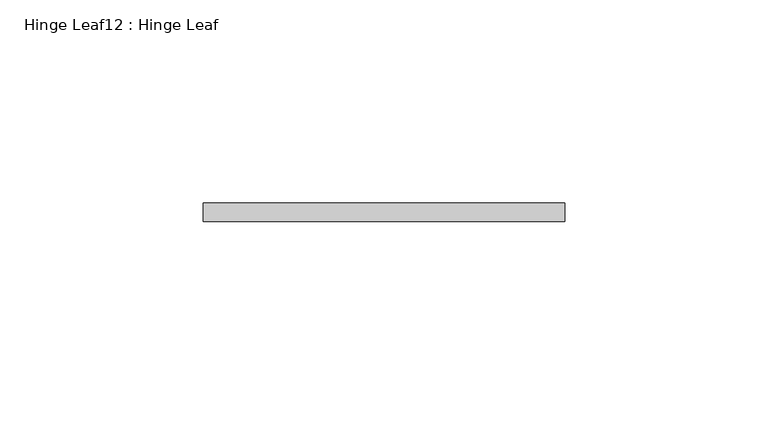
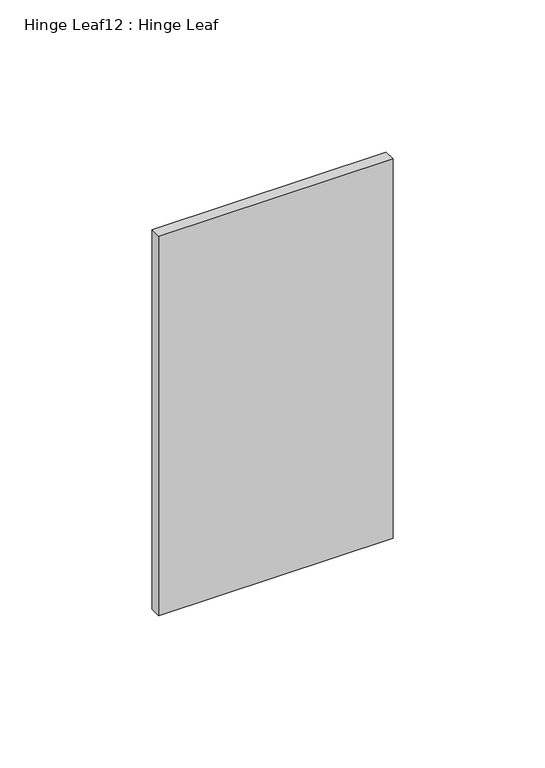
"""IFC4 building model written with IfcOpenShell, lengths in millimetres: proxy geometry, Hinge Leaf12 : Hinge Leaf."""

import ifcopenshell
import ifcopenshell.guid

model = None  # the IFC model being written
_history = None  # IfcOwnerHistory: only IFC2X3 demands one
_inside = {}  # id of a spatial element -> (the spatial element, [elements in it])
_under = {}  # id of a project, library or spatial element -> (it, [spatial elements below it])
_declared = {}  # id of a project -> (the project, [libraries it declares])
_typed = {}  # id of a type object -> (the type object, [elements of that type])
_made_of = {}  # id of a material, layer set ... -> (it, [elements and type objects made of it])


def new_model(schema):
    """Start an empty IFC model of exactly this schema.

    Asked for "IFC4X3", IfcOpenShell would pick the latest addendum, in which some entities
    have other attributes; the version numbers below select the first issue.
    IFC2X3 requires an IfcOwnerHistory on every rooted entity: one is made here for all.
    """
    global model, _history
    if schema == "IFC4X3":
        model = ifcopenshell.file(schema_version=(4, 3, 0, 0))
    else:
        model = ifcopenshell.file(schema=schema)
    _inside.clear()
    _under.clear()
    _declared.clear()
    _typed.clear()
    _made_of.clear()
    _history = None
    if model.schema == "IFC2X3":
        org = make("IfcOrganization", Name="unknown")
        user = make(
            "IfcPersonAndOrganization",
            ThePerson=make("IfcPerson", FamilyName="unknown"),
            TheOrganization=org,
        )
        app = make(
            "IfcApplication",
            ApplicationDeveloper=org,
            Version="unknown",
            ApplicationFullName="unknown",
            ApplicationIdentifier="unknown",
        )
        _history = make(
            "IfcOwnerHistory",
            OwningUser=user,
            OwningApplication=app,
            ChangeAction="ADDED",
            CreationDate=0,
        )
    return model


def make(cls, **values):
    """One entity of the class cls with the attributes given. An attribute that is None is left unset."""
    return model.create_entity(
        cls, **{name: value for name, value in values.items() if value is not None}
    )


def rooted(cls, **values):
    """An entity with a GlobalId (a new one), such as an element, a storey or a relation."""
    return make(cls, GlobalId=ifcopenshell.guid.new(), OwnerHistory=_history, **values)


def si_unit(unit_type, name, prefix=None):
    """IfcSIUnit, for example si_unit("LENGTHUNIT", "METRE", prefix="MILLI")."""
    return make("IfcSIUnit", UnitType=unit_type, Prefix=prefix, Name=name)


def assignment(units):
    """IfcUnitAssignment: the units of a project."""
    return None if units is None else make("IfcUnitAssignment", Units=units)


def point(xyz):
    """IfcCartesianPoint."""
    return None if xyz is None else make("IfcCartesianPoint", Coordinates=xyz)


def direction(xyz):
    """IfcDirection."""
    return None if xyz is None else make("IfcDirection", DirectionRatios=xyz)


def frame(location, z_axis=None, x_axis=None):
    """IfcAxis2Placement3D, a coordinate frame: its origin and axes. An axis left out is left unset."""
    return make(
        "IfcAxis2Placement3D",
        Location=point(location),
        Axis=direction(z_axis),
        RefDirection=direction(x_axis),
    )


def origin():
    """The frame at (0, 0, 0) with its axes left unset."""
    return frame((0.0, 0.0, 0.0))


def place(relative_to, where):
    """IfcLocalPlacement: puts the frame where relative to a parent placement (None: the world)."""
    return make(
        "IfcLocalPlacement", PlacementRelTo=relative_to, RelativePlacement=where
    )


def context(
    kind, dimensions, precision=None, world=None, true_north=None, identifier=None
):
    """IfcGeometricRepresentationContext, for example the 3D "Model" context."""
    return make(
        "IfcGeometricRepresentationContext",
        ContextIdentifier=identifier,
        ContextType=kind,
        CoordinateSpaceDimension=dimensions,
        Precision=precision,
        WorldCoordinateSystem=world,
        TrueNorth=true_north,
    )


def project(units=None, contexts=None):
    """IfcProject with its units and contexts."""
    return rooted(
        "IfcProject",
        Name="project",
        RepresentationContexts=contexts,
        UnitsInContext=assignment(units),
    )


def spatial(cls, under=None, at=None, **own):
    """A site, building, storey or space (cls), placed at a placement, below another one or the project."""
    s = rooted(cls, ObjectPlacement=at, **own)
    if under is not None:
        _under.setdefault(under.id(), (under, []))[1].append(s)
    return s


def polyline(points):
    """IfcPolyline through the points."""
    return make("IfcPolyline", Points=[point(p) for p in points])


def outline(outer, holes=None, kind="AREA"):
    """IfcArbitraryClosedProfileDef: a profile drawn as a closed curve; with holes, ...WithVoids."""
    if holes is None:
        return make("IfcArbitraryClosedProfileDef", ProfileType=kind, OuterCurve=outer)
    return make(
        "IfcArbitraryProfileDefWithVoids",
        ProfileType=kind,
        OuterCurve=outer,
        InnerCurves=holes,
    )


def extrude(swept, where, along, depth):
    """IfcExtrudedAreaSolid: the profile swept, set in the frame where, extruded along a direction by depth."""
    return make(
        "IfcExtrudedAreaSolid",
        SweptArea=swept,
        Position=where,
        ExtrudedDirection=direction(along),
        Depth=depth,
    )


def shape(context_of_items, identifier, shape_type, items):
    """IfcShapeRepresentation: the items that make up one representation, for example the "Body"."""
    return make(
        "IfcShapeRepresentation",
        ContextOfItems=context_of_items,
        RepresentationIdentifier=identifier,
        RepresentationType=shape_type,
        Items=items,
    )


def source(mapping_origin, context_of_items, identifier, shape_type, items):
    """IfcRepresentationMap: a shape defined once, which mapped items show again and again."""
    return make(
        "IfcRepresentationMap",
        MappingOrigin=mapping_origin,
        MappedRepresentation=shape(context_of_items, identifier, shape_type, items),
    )


def transform(
    local_origin,
    x_axis=None,
    y_axis=None,
    z_axis=None,
    scale=None,
    scale2=None,
    scale3=None,
    uniform=True,
):
    """IfcCartesianTransformationOperator3D, or its non-uniform kind. x_axis, y_axis, z_axis: its Axis1, 2, 3."""
    if uniform:
        return make(
            "IfcCartesianTransformationOperator3D",
            Axis1=direction(x_axis),
            Axis2=direction(y_axis),
            LocalOrigin=point(local_origin),
            Scale=scale,
            Axis3=direction(z_axis),
        )
    return make(
        "IfcCartesianTransformationOperator3DnonUniform",
        Axis1=direction(x_axis),
        Axis2=direction(y_axis),
        LocalOrigin=point(local_origin),
        Scale=scale,
        Axis3=direction(z_axis),
        Scale2=scale2,
        Scale3=scale3,
    )


def mapped(mapping_source, mapping_target):
    """IfcMappedItem: shows the shape of a source again, moved by a transform."""
    return make(
        "IfcMappedItem", MappingSource=mapping_source, MappingTarget=mapping_target
    )


def made_of(thing, what):
    """Note that an element or type object is made of a material, layer set ...; save() writes the relation."""
    if what is not None:
        _made_of.setdefault(what.id(), (what, []))[1].append(thing)
    return thing


def element(
    cls,
    number,
    at=None,
    inside=None,
    cuts=None,
    type_object=None,
    material=None,
    context=None,
    identifier="Body",
    shape_type=None,
    held_by="IfcProductDefinitionShape",
    body=None,
    shapes=None,
    **own,
):
    """One element of the class cls, such as IfcWall. Its Tag is "e" and its number.

    at: its placement. inside: the storey or other place that contains it. cuts: it is an
    opening in that element (IfcRelVoidsElement). A single representation is given by context,
    identifier, shape_type and body (its items); several are given by shapes. held_by: the class
    of the entity that holds the representations. save() writes the other relations.
    """
    e = rooted(cls, Tag="e%d" % number, ObjectPlacement=at, **own)
    if body is not None:
        shapes = [shape(context, identifier, shape_type, body)]
    if shapes is not None:
        e.Representation = make(held_by, Representations=shapes)
    if inside is not None:
        _inside.setdefault(inside.id(), (inside, []))[1].append(e)
    if cuts is not None:
        rooted(
            "IfcRelVoidsElement", RelatingBuildingElement=cuts, RelatedOpeningElement=e
        )
    if type_object is not None:
        _typed.setdefault(type_object.id(), (type_object, []))[1].append(e)
    return made_of(e, material)


def aggregate(whole, parts):
    """IfcRelAggregates: a whole, such as a stair, and the parts it consists of."""
    return rooted("IfcRelAggregates", RelatingObject=whole, RelatedObjects=parts)


def save(model, path):
    """Write the relations noted so far, then the file.

    IfcRelAggregates (storeys below a building ...), IfcRelContainedInSpatialStructure (elements
    in a storey), IfcRelDefinesByType, IfcRelAssociatesMaterial and IfcRelDeclares: one each for
    every whole, place, type object, material and project.
    """
    for whole, parts in _under.values():
        aggregate(whole, parts)
    for where, things in _inside.values():
        rooted(
            "IfcRelContainedInSpatialStructure",
            RelatedElements=things,
            RelatingStructure=where,
        )
    for kind, things in _typed.values():
        rooted("IfcRelDefinesByType", RelatedObjects=things, RelatingType=kind)
    for what, things in _made_of.values():
        rooted("IfcRelAssociatesMaterial", RelatedObjects=things, RelatingMaterial=what)
    for by, libraries in _declared.values():
        rooted("IfcRelDeclares", RelatingContext=by, RelatedDefinitions=libraries)
    model.write(path)


def hinge_leaf12_hinge_leaf_05c7f3a5(model_context):
    return source(origin(), model_context, "Body", "SweptSolid", [
        extrude(outline(polyline([(587327.7934739, -533980.5883841), (587327.7934739, -533976.0163841), (587416.6934739, -533976.0163841), (587416.6934739, -533980.5883841), (587327.7934739, -533980.5883841)])), frame((0.0, 0.0, 1123.95), z_axis=(0.0, 0.0, 1.0), x_axis=(1.0, 0.0, 0.0)), (0.0, 0.0, 1.0), 152.4),
    ])


if __name__ == "__main__":
    model = new_model("IFC4")
    model_context = context("Model", 3, world=origin())
    ifc_project = project(units=[si_unit("LENGTHUNIT", "METRE", prefix="MILLI")], contexts=[model_context])
    site = spatial("IfcSite", under=ifc_project)
    building = spatial("IfcBuilding", under=site)
    placement = place(None, origin())
    hinge_leaf12_hinge_leaf_shape = hinge_leaf12_hinge_leaf_05c7f3a5(model_context)
    element("IfcBuildingElementProxy", 1, Name="Hinge Leaf12 : Hinge Leaf", ObjectType="Hinge Leaf12 : Hinge Leaf", at=placement, inside=building, context=model_context, shape_type="MappedRepresentation", body=[
        mapped(hinge_leaf12_hinge_leaf_shape, transform((0.0, 0.0, 0.0), x_axis=(1.0, 0.0, 0.0), y_axis=(0.0, 1.0, 0.0), z_axis=(0.0, 0.0, 1.0))),
    ])
    save(model, "model.ifc")

# Revit data of these elements
# Element 1 (IfcBuildingElementProxy, "Hinge Leaf12 : Hinge Leaf")
#   Materials on its faces: "6\"X6\" WELD-ON STL BUTT HINGE"
# Materials
#   "6\"X6\" WELD-ON STL BUTT HINGE": class "Metal", colour RGB 189 187 185, transparency 0, Description = "Carbon steel", Cost = 0
